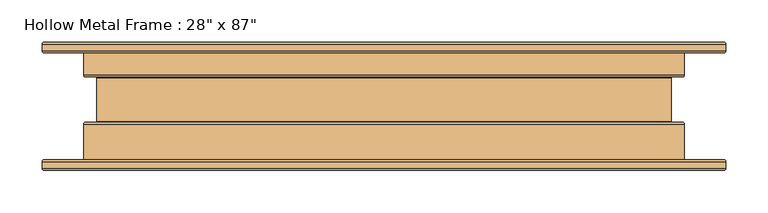
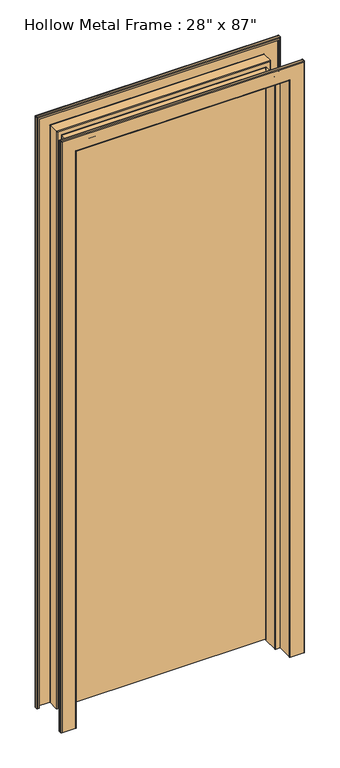
"""IFC4 building model written with IfcOpenShell, lengths in millimetres: door geometry."""

from ifc_helpers import new_model, si_unit, frame, origin, origin_with_axes, place, context, project, spatial, polyline, circle_curve, ellipse_curve, outline, extrude, source, transform, mapped, element, save
from ifc_brep_helpers import plane_surface, cylinder_surface, revolved_surface, advanced_brep


def door_6b69223f(model_context):
    return source(origin(), model_context, "Body", "SolidModel", [
        advanced_brep(
        [(-403.82825, -63.5635, 0.0), (-398.4625, -63.5635, 0.0), (-398.4625, -65.11925, 0.0), (-403.82825, -65.11925, 0.0), (-404.84425, -66.13525, 0.0), (-404.84425, -73.66, 0.0), (-403.82825, -74.676, 0.0), (-358.17175, -74.676, 0.0), (-357.15575, -73.66, 0.0), (-357.15575, -21.68525, 0.0), (-354.584, -19.1135, 0.0), (-342.29675, -19.1135, 0.0), (-341.28075, -18.0975, 0.0), (-341.28075, 33.6931, 0.0), (-342.29675, 34.7091, 0.0), (-354.584, 34.7091, 0.0), (-357.15575, 37.28085, 0.0), (-357.15575, 73.5965, 0.0), (-358.17175, 74.6125, 0.0), (-403.82825, 74.6125, 0.0), (-404.84425, 73.5965, 0.0), (-404.84425, 66.07175, 0.0), (-403.82825, 65.05575, 0.0), (-398.4625, 65.05575, 0.0), (-398.4625, 63.5, 0.0), (-403.82825, 63.5, 0.0), (-406.4, 66.07175, 0.0), (-406.4, 73.5965, 0.0), (-403.82825, 76.16825, 0.0), (-358.17175, 76.16825, 0.0), (-355.6, 73.5965, 0.0), (-355.6, 37.28085, 0.0), (-354.584, 36.26485, 0.0), (-342.29675, 36.26485, 0.0), (-339.725, 33.6931, 0.0), (-339.725, -18.0975, 0.0), (-342.29675, -20.66925, 0.0), (-354.584, -20.66925, 0.0), (-355.6, -21.68525, 0.0), (-355.6, -73.66, 0.0), (-358.17175, -76.23175, 0.0), (-403.82825, -76.23175, 0.0), (-406.4, -73.66, 0.0), (-406.4, -66.13525, 0.0), (-406.4, -66.13525, 2082.8000001), (-403.82825, -63.5635, 2080.2282501), (-406.4, -73.66, 2082.8000001), (-403.82825, -76.23175, 2080.2282501), (-358.17175, -76.23175, 2034.5717501), (358.17175, -76.23175, 2034.5717501), (358.17175, -76.23175, 0.0), (403.82825, -76.23175, 0.0), (403.82825, -76.23175, 2080.2282501), (-355.6, -73.66, 2032.0000001), (-355.6, -21.68525, 2032.0000001), (-354.584, -20.66925, 2030.9840001), (-342.29675, -20.66925, 2018.6967501), (342.29675, -20.66925, 2018.6967501), (342.29675, -20.66925, 0.0), (354.584, -20.66925, 0.0), (354.584, -20.66925, 2030.9840001), (-339.725, -18.0975, 2016.1250001), (-339.725, 33.6931, 2016.1250001), (-342.29675, 36.26485, 2018.6967501), (-354.584, 36.26485, 2030.9840001), (354.584, 36.26485, 2030.9840001), (354.584, 36.26485, 0.0), (342.29675, 36.26485, 0.0), (342.29675, 36.26485, 2018.6967501), (-355.6, 37.28085, 2032.0000001), (-355.6, 73.5965, 2032.0000001), (-358.17175, 76.16825, 2034.5717501), (-403.82825, 76.16825, 2080.2282501), (403.82825, 76.16825, 2080.2282501), (403.82825, 76.16825, 0.0), (358.17175, 76.16825, 0.0), (358.17175, 76.16825, 2034.5717501), (-406.4, 73.5965, 2082.8000001), (-406.4, 66.07175, 2082.8000001), (-403.82825, 63.5, 2080.2282501), (-398.4625, 63.5, 2074.8625001), (398.4625, 63.5, 2074.8625001), (398.4625, 63.5, 0.0), (403.82825, 63.5, 0.0), (403.82825, 63.5, 2080.2282501), (-398.4625, 65.05575, 2074.8625001), (-403.82825, 65.05575, 2080.2282501), (403.82825, 65.05575, 2080.2282501), (403.82825, 65.05575, 0.0), (398.4625, 65.05575, 0.0), (398.4625, 65.05575, 2074.8625001), (-404.84425, 66.07175, 2081.2442501), (-404.84425, 73.5965, 2081.2442501), (-403.82825, 74.6125, 2080.2282501), (-358.17175, 74.6125, 2034.5717501), (358.17175, 74.6125, 2034.5717501), (358.17175, 74.6125, 0.0), (403.82825, 74.6125, 0.0), (403.82825, 74.6125, 2080.2282501), (-357.15575, 73.5965, 2033.5557501), (-357.15575, 37.28085, 2033.5557501), (-354.584, 34.7091, 2030.9840001), (-342.29675, 34.7091, 2018.6967501), (342.29675, 34.7091, 2018.6967501), (342.29675, 34.7091, 0.0), (354.584, 34.7091, 0.0), (354.584, 34.7091, 2030.9840001), (-341.28075, 33.6931, 2017.6807501), (-341.28075, -18.0975, 2017.6807501), (-342.29675, -19.1135, 2018.6967501), (-354.584, -19.1135, 2030.9840001), (354.584, -19.1135, 2030.9840001), (354.584, -19.1135, 0.0), (342.29675, -19.1135, 0.0), (342.29675, -19.1135, 2018.6967501), (-357.15575, -21.68525, 2033.5557501), (-357.15575, -73.66, 2033.5557501), (-358.17175, -74.676, 2034.5717501), (-403.82825, -74.676, 2080.2282501), (403.82825, -74.676, 2080.2282501), (403.82825, -74.676, 0.0), (358.17175, -74.676, 0.0), (358.17175, -74.676, 2034.5717501), (-404.84425, -73.66, 2081.2442501), (-404.84425, -66.13525, 2081.2442501), (-403.82825, -65.11925, 2080.2282501), (-398.4625, -65.11925, 2074.8625001), (398.4625, -65.11925, 2074.8625001), (398.4625, -65.11925, 0.0), (403.82825, -65.11925, 0.0), (403.82825, -65.11925, 2080.2282501), (-398.4625, -63.5635, 2074.8625001), (403.82825, -63.5635, 2080.2282501), (403.82825, -63.5635, 0.0), (398.4625, -63.5635, 0.0), (398.4625, -63.5635, 2074.8625001), (406.4, -66.13525, 2082.8000001), (406.4, -73.66, 2082.8000001), (355.6, -73.66, 2032.0000001), (355.6, -21.68525, 2032.0000001), (339.725, -18.0975, 2016.1250001), (339.725, 33.6931, 2016.1250001), (355.6, 37.28085, 2032.0000001), (355.6, 73.5965, 2032.0000001), (406.4, 73.5965, 2082.8000001), (406.4, 66.07175, 2082.8000001), (404.84425, 66.07175, 2081.2442501), (404.84425, 73.5965, 2081.2442501), (357.15575, 73.5965, 2033.5557501), (357.15575, 37.28085, 2033.5557501), (341.28075, 33.6931, 2017.6807501), (341.28075, -18.0975, 2017.6807501), (357.15575, -21.68525, 2033.5557501), (357.15575, -73.66, 2033.5557501), (404.84425, -73.66, 2081.2442501), (404.84425, -66.13525, 2081.2442501), (406.4, -66.13525, 0.0), (406.4, -73.66, 0.0), (355.6, -73.66, 0.0), (355.6, -21.68525, 0.0), (339.725, -18.0975, 0.0), (339.725, 33.6931, 0.0), (355.6, 37.28085, 0.0), (355.6, 73.5965, 0.0), (406.4, 73.5965, 0.0), (406.4, 66.07175, 0.0), (404.84425, 66.07175, 0.0), (404.84425, 73.5965, 0.0), (357.15575, 73.5965, 0.0), (357.15575, 37.28085, 0.0), (341.28075, 33.6931, 0.0), (341.28075, -18.0975, 0.0), (357.15575, -21.68525, 0.0), (357.15575, -73.66, 0.0), (404.84425, -73.66, 0.0), (404.84425, -66.13525, 0.0)],
        [
            (0, 1),
            (1, 2),
            (2, 3),
            (3, 4, circle_curve(frame((-403.82825, -66.13525, 0.0), z_axis=(0.0, 0.0, 1.0), x_axis=(0.0, 1.0, 0.0)), 1.016)),
            (4, 5),
            (5, 6, circle_curve(frame((-403.82825, -73.66, 0.0), z_axis=(0.0, 0.0, 1.0), x_axis=(0.0, 1.0, 0.0)), 1.016)),
            (6, 7),
            (7, 8, circle_curve(frame((-358.17175, -73.66, 0.0), z_axis=(0.0, 0.0, 1.0), x_axis=(0.0, 1.0, 0.0)), 1.016)),
            (8, 9),
            (9, 10, circle_curve(frame((-354.584, -21.68525, 0.0), z_axis=(0.0, 0.0, -1.0), x_axis=(0.0, 1.0, 0.0)), 2.57175)),
            (10, 11),
            (11, 12, circle_curve(frame((-342.29675, -18.0975, 0.0), z_axis=(0.0, 0.0, 1.0), x_axis=(0.0, 1.0, 0.0)), 1.016)),
            (12, 13),
            (13, 14, circle_curve(frame((-342.29675, 33.6931, 0.0), z_axis=(0.0, 0.0, 1.0), x_axis=(0.0, 1.0, 0.0)), 1.016)),
            (14, 15),
            (15, 16, circle_curve(frame((-354.584, 37.28085, 0.0), z_axis=(0.0, 0.0, -1.0), x_axis=(0.0, 1.0, 0.0)), 2.57175)),
            (16, 17),
            (17, 18, circle_curve(frame((-358.17175, 73.5965, 0.0), z_axis=(0.0, 0.0, 1.0), x_axis=(0.0, 1.0, 0.0)), 1.016)),
            (18, 19),
            (19, 20, circle_curve(frame((-403.82825, 73.5965, 0.0), z_axis=(0.0, 0.0, 1.0), x_axis=(0.0, 1.0, 0.0)), 1.016)),
            (20, 21),
            (21, 22, circle_curve(frame((-403.82825, 66.07175, 0.0), z_axis=(0.0, 0.0, 1.0), x_axis=(0.0, 1.0, 0.0)), 1.016)),
            (22, 23),
            (23, 24),
            (24, 25),
            (25, 26, circle_curve(frame((-403.82825, 66.07175, 0.0), z_axis=(0.0, 0.0, -1.0), x_axis=(0.0, 1.0, 0.0)), 2.57175)),
            (26, 27),
            (27, 28, circle_curve(frame((-403.82825, 73.5965, 0.0), z_axis=(0.0, 0.0, -1.0), x_axis=(0.0, 1.0, 0.0)), 2.57175)),
            (28, 29),
            (29, 30, circle_curve(frame((-358.17175, 73.5965, 0.0), z_axis=(0.0, 0.0, -1.0), x_axis=(0.0, 1.0, 0.0)), 2.57175)),
            (30, 31),
            (31, 32, circle_curve(frame((-354.584, 37.28085, 0.0), z_axis=(0.0, 0.0, 1.0), x_axis=(0.0, 1.0, 0.0)), 1.016)),
            (32, 33),
            (33, 34, circle_curve(frame((-342.29675, 33.6931, 0.0), z_axis=(0.0, 0.0, -1.0), x_axis=(0.0, 1.0, 0.0)), 2.57175)),
            (34, 35),
            (35, 36, circle_curve(frame((-342.29675, -18.0975, 0.0), z_axis=(0.0, 0.0, -1.0), x_axis=(0.0, 1.0, 0.0)), 2.57175)),
            (36, 37),
            (37, 38, circle_curve(frame((-354.584, -21.68525, 0.0), z_axis=(0.0, 0.0, 1.0), x_axis=(0.0, 1.0, 0.0)), 1.016)),
            (38, 39),
            (39, 40, circle_curve(frame((-358.17175, -73.66, 0.0), z_axis=(0.0, 0.0, -1.0), x_axis=(0.0, 1.0, 0.0)), 2.57175)),
            (40, 41),
            (41, 42, circle_curve(frame((-403.82825, -73.66, 0.0), z_axis=(0.0, 0.0, -1.0), x_axis=(0.0, 1.0, 0.0)), 2.57175)),
            (42, 43),
            (43, 0, circle_curve(frame((-403.82825, -66.13525, 0.0), z_axis=(0.0, 0.0, -1.0), x_axis=(0.0, 1.0, 0.0)), 2.57175)),
            (43, 44),
            (44, 45, ellipse_curve(frame((-403.82825, -66.13525, 2080.2282501), z_axis=(-0.7071067811865475, 0.0, -0.7071067811865475), x_axis=(0.7071067811865474, 0.0, -0.7071067811865476)), 3.6370037, 2.57175)),
            (45, 0),
            (42, 46),
            (46, 44),
            (41, 47),
            (47, 46, ellipse_curve(frame((-403.82825, -73.66, 2080.2282501), z_axis=(-0.7071067811865475, 0.0, -0.7071067811865475), x_axis=(0.7071067811865474, 0.0, -0.7071067811865476)), 3.6370037, 2.57175)),
            (40, 48),
            (48, 49),
            (49, 50),
            (50, 51),
            (51, 52),
            (52, 47),
            (39, 53),
            (53, 48, ellipse_curve(frame((-358.17175, -73.66, 2034.5717501), z_axis=(-0.7071067811865475, 0.0, -0.7071067811865475), x_axis=(0.7071067811865474, 0.0, -0.7071067811865476)), 3.6370037, 2.57175)),
            (38, 54),
            (54, 53),
            (37, 55),
            (55, 54, ellipse_curve(frame((-354.584, -21.68525, 2030.9840001), z_axis=(0.7071067811865475, 0.0, 0.7071067811865475), x_axis=(-0.7071067811865474, 0.0, 0.7071067811865476)), 1.436841, 1.016)),
            (36, 56),
            (56, 57),
            (57, 58),
            (58, 59),
            (59, 60),
            (60, 55),
            (35, 61),
            (61, 56, ellipse_curve(frame((-342.29675, -18.0975, 2018.6967501), z_axis=(-0.7071067811865475, 0.0, -0.7071067811865475), x_axis=(0.7071067811865474, 0.0, -0.7071067811865476)), 3.6370037, 2.57175)),
            (34, 62),
            (62, 61),
            (33, 63),
            (63, 62, ellipse_curve(frame((-342.29675, 33.6931, 2018.6967501), z_axis=(-0.7071067811865475, 0.0, -0.7071067811865475), x_axis=(0.7071067811865474, 0.0, -0.7071067811865476)), 3.6370037, 2.57175)),
            (32, 64),
            (64, 65),
            (65, 66),
            (66, 67),
            (67, 68),
            (68, 63),
            (31, 69),
            (69, 64, ellipse_curve(frame((-354.584, 37.28085, 2030.9840001), z_axis=(0.7071067811865475, 0.0, 0.7071067811865475), x_axis=(-0.7071067811865474, 0.0, 0.7071067811865476)), 1.436841, 1.016)),
            (30, 70),
            (70, 69),
            (29, 71),
            (71, 70, ellipse_curve(frame((-358.17175, 73.5965, 2034.5717501), z_axis=(-0.7071067811865475, 0.0, -0.7071067811865475), x_axis=(0.7071067811865474, 0.0, -0.7071067811865476)), 3.6370037, 2.57175)),
            (28, 72),
            (72, 73),
            (73, 74),
            (74, 75),
            (75, 76),
            (76, 71),
            (27, 77),
            (77, 72, ellipse_curve(frame((-403.82825, 73.5965, 2080.2282501), z_axis=(-0.7071067811865475, 0.0, -0.7071067811865475), x_axis=(0.7071067811865474, 0.0, -0.7071067811865476)), 3.6370037, 2.57175)),
            (26, 78),
            (78, 77),
            (25, 79),
            (79, 78, ellipse_curve(frame((-403.82825, 66.07175, 2080.2282501), z_axis=(-0.7071067811865475, 0.0, -0.7071067811865475), x_axis=(0.7071067811865474, 0.0, -0.7071067811865476)), 3.6370037, 2.57175)),
            (24, 80),
            (80, 81),
            (81, 82),
            (82, 83),
            (83, 84),
            (84, 79),
            (23, 85),
            (85, 80),
            (22, 86),
            (86, 87),
            (87, 88),
            (88, 89),
            (89, 90),
            (90, 85),
            (21, 91),
            (91, 86, ellipse_curve(frame((-403.82825, 66.07175, 2080.2282501), z_axis=(0.7071067811865475, 0.0, 0.7071067811865475), x_axis=(-0.7071067811865474, 0.0, 0.7071067811865476)), 1.436841, 1.016)),
            (20, 92),
            (92, 91),
            (19, 93),
            (93, 92, ellipse_curve(frame((-403.82825, 73.5965, 2080.2282501), z_axis=(0.7071067811865475, 0.0, 0.7071067811865475), x_axis=(-0.7071067811865474, 0.0, 0.7071067811865476)), 1.436841, 1.016)),
            (18, 94),
            (94, 95),
            (95, 96),
            (96, 97),
            (97, 98),
            (98, 93),
            (17, 99),
            (99, 94, ellipse_curve(frame((-358.17175, 73.5965, 2034.5717501), z_axis=(0.7071067811865475, 0.0, 0.7071067811865475), x_axis=(-0.7071067811865474, 0.0, 0.7071067811865476)), 1.436841, 1.016)),
            (16, 100),
            (100, 99),
            (15, 101),
            (101, 100, ellipse_curve(frame((-354.584, 37.28085, 2030.9840001), z_axis=(-0.7071067811865475, 0.0, -0.7071067811865475), x_axis=(0.7071067811865474, 0.0, -0.7071067811865476)), 3.6370037, 2.57175)),
            (14, 102),
            (102, 103),
            (103, 104),
            (104, 105),
            (105, 106),
            (106, 101),
            (13, 107),
            (107, 102, ellipse_curve(frame((-342.29675, 33.6931, 2018.6967501), z_axis=(0.7071067811865475, 0.0, 0.7071067811865475), x_axis=(-0.7071067811865474, 0.0, 0.7071067811865476)), 1.436841, 1.016)),
            (12, 108),
            (108, 107),
            (11, 109),
            (109, 108, ellipse_curve(frame((-342.29675, -18.0975, 2018.6967501), z_axis=(0.7071067811865475, 0.0, 0.7071067811865475), x_axis=(-0.7071067811865474, 0.0, 0.7071067811865476)), 1.436841, 1.016)),
            (10, 110),
            (110, 111),
            (111, 112),
            (112, 113),
            (113, 114),
            (114, 109),
            (9, 115),
            (115, 110, ellipse_curve(frame((-354.584, -21.68525, 2030.9840001), z_axis=(-0.7071067811865475, 0.0, -0.7071067811865475), x_axis=(0.7071067811865474, 0.0, -0.7071067811865476)), 3.6370037, 2.57175)),
            (8, 116),
            (116, 115),
            (7, 117),
            (117, 116, ellipse_curve(frame((-358.17175, -73.66, 2034.5717501), z_axis=(0.7071067811865475, 0.0, 0.7071067811865475), x_axis=(-0.7071067811865474, 0.0, 0.7071067811865476)), 1.436841, 1.016)),
            (6, 118),
            (118, 119),
            (119, 120),
            (120, 121),
            (121, 122),
            (122, 117),
            (5, 123),
            (123, 118, ellipse_curve(frame((-403.82825, -73.66, 2080.2282501), z_axis=(0.7071067811865475, 0.0, 0.7071067811865475), x_axis=(-0.7071067811865474, 0.0, 0.7071067811865476)), 1.436841, 1.016)),
            (4, 124),
            (124, 123),
            (3, 125),
            (125, 124, ellipse_curve(frame((-403.82825, -66.13525, 2080.2282501), z_axis=(0.7071067811865475, 0.0, 0.7071067811865475), x_axis=(-0.7071067811865474, 0.0, 0.7071067811865476)), 1.436841, 1.016)),
            (2, 126),
            (126, 127),
            (127, 128),
            (128, 129),
            (129, 130),
            (130, 125),
            (1, 131),
            (131, 126),
            (45, 132),
            (132, 133),
            (133, 134),
            (134, 135),
            (135, 131),
            (44, 136),
            (136, 132, ellipse_curve(frame((403.82825, -66.13525, 2080.2282501), z_axis=(-0.7071067811865475, 0.0, 0.7071067811865475), x_axis=(-0.7071067811865476, 0.0, -0.7071067811865474)), 3.6370037, 2.57175)),
            (46, 137),
            (137, 136),
            (52, 137, ellipse_curve(frame((403.82825, -73.66, 2080.2282501), z_axis=(-0.7071067811865475, 0.0, 0.7071067811865475), x_axis=(-0.7071067811865476, 0.0, -0.7071067811865474)), 3.6370037, 2.57175)),
            (53, 138),
            (138, 49, ellipse_curve(frame((358.17175, -73.66, 2034.5717501), z_axis=(-0.7071067811865475, 0.0, 0.7071067811865475), x_axis=(-0.7071067811865476, 0.0, -0.7071067811865474)), 3.6370037, 2.57175)),
            (54, 139),
            (139, 138),
            (60, 139, ellipse_curve(frame((354.584, -21.68525, 2030.9840001), z_axis=(0.7071067811865475, 0.0, -0.7071067811865475), x_axis=(0.7071067811865476, 0.0, 0.7071067811865474)), 1.436841, 1.016)),
            (61, 140),
            (140, 57, ellipse_curve(frame((342.29675, -18.0975, 2018.6967501), z_axis=(-0.7071067811865475, 0.0, 0.7071067811865475), x_axis=(-0.7071067811865476, 0.0, -0.7071067811865474)), 3.6370037, 2.57175)),
            (62, 141),
            (141, 140),
            (68, 141, ellipse_curve(frame((342.29675, 33.6931, 2018.6967501), z_axis=(-0.7071067811865475, 0.0, 0.7071067811865475), x_axis=(-0.7071067811865476, 0.0, -0.7071067811865474)), 3.6370037, 2.57175)),
            (69, 142),
            (142, 65, ellipse_curve(frame((354.584, 37.28085, 2030.9840001), z_axis=(0.7071067811865475, 0.0, -0.7071067811865475), x_axis=(0.7071067811865476, 0.0, 0.7071067811865474)), 1.436841, 1.016)),
            (70, 143),
            (143, 142),
            (76, 143, ellipse_curve(frame((358.17175, 73.5965, 2034.5717501), z_axis=(-0.7071067811865475, 0.0, 0.7071067811865475), x_axis=(-0.7071067811865476, 0.0, -0.7071067811865474)), 3.6370037, 2.57175)),
            (77, 144),
            (144, 73, ellipse_curve(frame((403.82825, 73.5965, 2080.2282501), z_axis=(-0.7071067811865475, 0.0, 0.7071067811865475), x_axis=(-0.7071067811865476, 0.0, -0.7071067811865474)), 3.6370037, 2.57175)),
            (78, 145),
            (145, 144),
            (84, 145, ellipse_curve(frame((403.82825, 66.07175, 2080.2282501), z_axis=(-0.7071067811865475, 0.0, 0.7071067811865475), x_axis=(-0.7071067811865476, 0.0, -0.7071067811865474)), 3.6370037, 2.57175)),
            (90, 81),
            (91, 146),
            (146, 87, ellipse_curve(frame((403.82825, 66.07175, 2080.2282501), z_axis=(0.7071067811865475, 0.0, -0.7071067811865475), x_axis=(0.7071067811865476, 0.0, 0.7071067811865474)), 1.436841, 1.016)),
            (92, 147),
            (147, 146),
            (98, 147, ellipse_curve(frame((403.82825, 73.5965, 2080.2282501), z_axis=(0.7071067811865475, 0.0, -0.7071067811865475), x_axis=(0.7071067811865476, 0.0, 0.7071067811865474)), 1.436841, 1.016)),
            (99, 148),
            (148, 95, ellipse_curve(frame((358.17175, 73.5965, 2034.5717501), z_axis=(0.7071067811865475, 0.0, -0.7071067811865475), x_axis=(0.7071067811865476, 0.0, 0.7071067811865474)), 1.436841, 1.016)),
            (100, 149),
            (149, 148),
            (106, 149, ellipse_curve(frame((354.584, 37.28085, 2030.9840001), z_axis=(-0.7071067811865475, 0.0, 0.7071067811865475), x_axis=(-0.7071067811865476, 0.0, -0.7071067811865474)), 3.6370037, 2.57175)),
            (107, 150),
            (150, 103, ellipse_curve(frame((342.29675, 33.6931, 2018.6967501), z_axis=(0.7071067811865475, 0.0, -0.7071067811865475), x_axis=(0.7071067811865476, 0.0, 0.7071067811865474)), 1.436841, 1.016)),
            (108, 151),
            (151, 150),
            (114, 151, ellipse_curve(frame((342.29675, -18.0975, 2018.6967501), z_axis=(0.7071067811865475, 0.0, -0.7071067811865475), x_axis=(0.7071067811865476, 0.0, 0.7071067811865474)), 1.436841, 1.016)),
            (115, 152),
            (152, 111, ellipse_curve(frame((354.584, -21.68525, 2030.9840001), z_axis=(-0.7071067811865475, 0.0, 0.7071067811865475), x_axis=(-0.7071067811865476, 0.0, -0.7071067811865474)), 3.6370037, 2.57175)),
            (116, 153),
            (153, 152),
            (122, 153, ellipse_curve(frame((358.17175, -73.66, 2034.5717501), z_axis=(0.7071067811865475, 0.0, -0.7071067811865475), x_axis=(0.7071067811865476, 0.0, 0.7071067811865474)), 1.436841, 1.016)),
            (123, 154),
            (154, 119, ellipse_curve(frame((403.82825, -73.66, 2080.2282501), z_axis=(0.7071067811865475, 0.0, -0.7071067811865475), x_axis=(0.7071067811865476, 0.0, 0.7071067811865474)), 1.436841, 1.016)),
            (124, 155),
            (155, 154),
            (130, 155, ellipse_curve(frame((403.82825, -66.13525, 2080.2282501), z_axis=(0.7071067811865475, 0.0, -0.7071067811865475), x_axis=(0.7071067811865476, 0.0, 0.7071067811865474)), 1.436841, 1.016)),
            (135, 127),
            (133, 156, circle_curve(frame((403.82825, -66.13525, 0.0), z_axis=(0.0, 0.0, -1.0), x_axis=(0.0, 1.0, 0.0)), 2.57175)),
            (156, 157),
            (157, 51, circle_curve(frame((403.82825, -73.66, 0.0), z_axis=(0.0, 0.0, -1.0), x_axis=(0.0, 1.0, 0.0)), 2.57175)),
            (50, 158, circle_curve(frame((358.17175, -73.66, 0.0), z_axis=(0.0, 0.0, -1.0), x_axis=(0.0, 1.0, 0.0)), 2.57175)),
            (158, 159),
            (159, 59, circle_curve(frame((354.584, -21.68525, 0.0), z_axis=(0.0, 0.0, 1.0), x_axis=(0.0, 1.0, 0.0)), 1.016)),
            (58, 160, circle_curve(frame((342.29675, -18.0975, 0.0), z_axis=(0.0, 0.0, -1.0), x_axis=(0.0, 1.0, 0.0)), 2.57175)),
            (160, 161),
            (161, 67, circle_curve(frame((342.29675, 33.6931, 0.0), z_axis=(0.0, 0.0, -1.0), x_axis=(0.0, 1.0, 0.0)), 2.57175)),
            (66, 162, circle_curve(frame((354.584, 37.28085, 0.0), z_axis=(0.0, 0.0, 1.0), x_axis=(0.0, 1.0, 0.0)), 1.016)),
            (162, 163),
            (163, 75, circle_curve(frame((358.17175, 73.5965, 0.0), z_axis=(0.0, 0.0, -1.0), x_axis=(0.0, 1.0, 0.0)), 2.57175)),
            (74, 164, circle_curve(frame((403.82825, 73.5965, 0.0), z_axis=(0.0, 0.0, -1.0), x_axis=(0.0, 1.0, 0.0)), 2.57175)),
            (164, 165),
            (165, 83, circle_curve(frame((403.82825, 66.07175, 0.0), z_axis=(0.0, 0.0, -1.0), x_axis=(0.0, 1.0, 0.0)), 2.57175)),
            (82, 89),
            (88, 166, circle_curve(frame((403.82825, 66.07175, 0.0), z_axis=(0.0, 0.0, 1.0), x_axis=(0.0, 1.0, 0.0)), 1.016)),
            (166, 167),
            (167, 97, circle_curve(frame((403.82825, 73.5965, 0.0), z_axis=(0.0, 0.0, 1.0), x_axis=(0.0, 1.0, 0.0)), 1.016)),
            (96, 168, circle_curve(frame((358.17175, 73.5965, 0.0), z_axis=(0.0, 0.0, 1.0), x_axis=(0.0, 1.0, 0.0)), 1.016)),
            (168, 169),
            (169, 105, circle_curve(frame((354.584, 37.28085, 0.0), z_axis=(0.0, 0.0, -1.0), x_axis=(0.0, 1.0, 0.0)), 2.57175)),
            (104, 170, circle_curve(frame((342.29675, 33.6931, 0.0), z_axis=(0.0, 0.0, 1.0), x_axis=(0.0, 1.0, 0.0)), 1.016)),
            (170, 171),
            (171, 113, circle_curve(frame((342.29675, -18.0975, 0.0), z_axis=(0.0, 0.0, 1.0), x_axis=(0.0, 1.0, 0.0)), 1.016)),
            (112, 172, circle_curve(frame((354.584, -21.68525, 0.0), z_axis=(0.0, 0.0, -1.0), x_axis=(0.0, 1.0, 0.0)), 2.57175)),
            (172, 173),
            (173, 121, circle_curve(frame((358.17175, -73.66, 0.0), z_axis=(0.0, 0.0, 1.0), x_axis=(0.0, 1.0, 0.0)), 1.016)),
            (120, 174, circle_curve(frame((403.82825, -73.66, 0.0), z_axis=(0.0, 0.0, 1.0), x_axis=(0.0, 1.0, 0.0)), 1.016)),
            (174, 175),
            (175, 129, circle_curve(frame((403.82825, -66.13525, 0.0), z_axis=(0.0, 0.0, 1.0), x_axis=(0.0, 1.0, 0.0)), 1.016)),
            (128, 134),
            (136, 156),
            (137, 157),
            (138, 158),
            (139, 159),
            (140, 160),
            (141, 161),
            (142, 162),
            (143, 163),
            (144, 164),
            (145, 165),
            (146, 166),
            (147, 167),
            (148, 168),
            (149, 169),
            (150, 170),
            (151, 171),
            (152, 172),
            (153, 173),
            (154, 174),
            (155, 175),
        ],
        [
            plane_surface(frame((-366.7125, 63.5, 0.0), z_axis=(0.0, 0.0, -1.0), x_axis=(1.0, 0.0, 0.0))),
            cylinder_surface(frame((-403.82825, -66.13525, 0.0), z_axis=(0.0, 0.0, -1.0), x_axis=(0.0, 1.0, 0.0)), 2.57175),
            plane_surface(frame((-406.4, -66.13525, 0.0), z_axis=(-1.0, 0.0, 0.0), x_axis=(0.0, 0.0, 1.0))),
            cylinder_surface(frame((-403.82825, -73.66, 0.0), z_axis=(0.0, 0.0, -1.0), x_axis=(0.0, 1.0, 0.0)), 2.57175),
            plane_surface(frame((-403.82825, -76.23175, 0.0), z_axis=(0.0, -1.0, 0.0), x_axis=(0.0, 0.0, 1.0))),
            cylinder_surface(frame((-358.17175, -73.66, 0.0), z_axis=(0.0, 0.0, -1.0), x_axis=(0.0, 1.0, 0.0)), 2.57175),
            plane_surface(frame((-355.6, -73.66, 0.0), z_axis=(1.0, 0.0, 0.0), x_axis=(0.0, 0.0, 1.0))),
            revolved_surface(polyline([(-354.584, -20.669249999999998, 2032.0000001145868), (-354.584, -20.669249999999998, 0.0)]), (-354.584, -21.68525, 0.0), (0.0, 0.0, 1.0)),
            plane_surface(frame((-354.584, -20.66925, 0.0), z_axis=(0.0, -1.0, 0.0), x_axis=(0.0, 0.0, 1.0))),
            cylinder_surface(frame((-342.29675, -18.0975, 0.0), z_axis=(0.0, 0.0, -1.0), x_axis=(0.0, 1.0, 0.0)), 2.57175),
            plane_surface(frame((-339.725, -18.0975, 0.0), z_axis=(1.0, 0.0, 0.0), x_axis=(0.0, 0.0, 1.0))),
            cylinder_surface(frame((-342.29675, 33.6931, 0.0), z_axis=(0.0, 0.0, -1.0), x_axis=(0.0, 1.0, 0.0)), 2.57175),
            plane_surface(frame((-342.29675, 36.26485, 0.0), z_axis=(0.0, 1.0, 0.0), x_axis=(0.0, 0.0, 1.0))),
            revolved_surface(polyline([(-354.584, 38.29685, 2032.0000001145868), (-354.584, 38.29685, 0.0)]), (-354.584, 37.28085, 0.0), (0.0, 0.0, 1.0)),
            plane_surface(frame((-355.6, 37.28085, 0.0), z_axis=(1.0, 0.0, 0.0), x_axis=(0.0, 0.0, 1.0))),
            cylinder_surface(frame((-358.17175, 73.5965, 0.0), z_axis=(0.0, 0.0, -1.0), x_axis=(0.0, 1.0, 0.0)), 2.57175),
            plane_surface(frame((-358.17175, 76.16825, 0.0), z_axis=(0.0, 1.0, 0.0), x_axis=(0.0, 0.0, 1.0))),
            cylinder_surface(frame((-403.82825, 73.5965, 0.0), z_axis=(0.0, 0.0, -1.0), x_axis=(0.0, 1.0, 0.0)), 2.57175),
            plane_surface(frame((-406.4, 73.5965, 0.0), z_axis=(-1.0, 0.0, 0.0), x_axis=(0.0, 0.0, 1.0))),
            cylinder_surface(frame((-403.82825, 66.07175, 0.0), z_axis=(0.0, 0.0, -1.0), x_axis=(0.0, 1.0, 0.0)), 2.57175),
            plane_surface(frame((-403.82825, 63.5, 0.0), z_axis=(0.0, -1.0, 0.0), x_axis=(0.0, 0.0, 1.0))),
            plane_surface(frame((-398.4625, 63.5, 0.0), z_axis=(1.0, 0.0, 0.0), x_axis=(0.0, 0.0, 1.0))),
            plane_surface(frame((-398.4625, 65.05575, 0.0), z_axis=(0.0, 1.0, 0.0), x_axis=(0.0, 0.0, 1.0))),
            revolved_surface(polyline([(-403.82825, 67.08775, 2081.244250114587), (-403.82825, 67.08775, 0.0)]), (-403.82825, 66.07175, 0.0), (0.0, 0.0, 1.0)),
            plane_surface(frame((-404.84425, 66.07175, 0.0), z_axis=(1.0, 0.0, 0.0), x_axis=(0.0, 0.0, 1.0))),
            revolved_surface(polyline([(-403.82825, 74.61250000000001, 2081.244250114587), (-403.82825, 74.61250000000001, 0.0)]), (-403.82825, 73.5965, 0.0), (0.0, 0.0, 1.0)),
            plane_surface(frame((-403.82825, 74.6125, 0.0), z_axis=(0.0, -1.0, 0.0), x_axis=(0.0, 0.0, 1.0))),
            revolved_surface(polyline([(-358.17175, 74.61250000000001, 2035.5877501145867), (-358.17175, 74.61250000000001, 0.0)]), (-358.17175, 73.5965, 0.0), (0.0, 0.0, 1.0)),
            plane_surface(frame((-357.15575, 73.5965, 0.0), z_axis=(-1.0, 0.0, 0.0), x_axis=(0.0, 0.0, 1.0))),
            cylinder_surface(frame((-354.584, 37.28085, 0.0), z_axis=(0.0, 0.0, -1.0), x_axis=(0.0, 1.0, 0.0)), 2.57175),
            plane_surface(frame((-354.584, 34.7091, 0.0), z_axis=(0.0, -1.0, 0.0), x_axis=(0.0, 0.0, 1.0))),
            revolved_surface(polyline([(-342.29675, 34.7091, 2019.7127501145867), (-342.29675, 34.7091, 0.0)]), (-342.29675, 33.6931, 0.0), (0.0, 0.0, 1.0)),
            plane_surface(frame((-341.28075, 33.6931, 0.0), z_axis=(-1.0, 0.0, 0.0), x_axis=(0.0, 0.0, 1.0))),
            revolved_surface(polyline([(-342.29675, -17.0815, 2019.7127501145867), (-342.29675, -17.0815, 0.0)]), (-342.29675, -18.0975, 0.0), (0.0, 0.0, 1.0)),
            plane_surface(frame((-342.29675, -19.1135, 0.0), z_axis=(0.0, 1.0, 0.0), x_axis=(0.0, 0.0, 1.0))),
            cylinder_surface(frame((-354.584, -21.68525, 0.0), z_axis=(0.0, 0.0, -1.0), x_axis=(0.0, 1.0, 0.0)), 2.57175),
            plane_surface(frame((-357.15575, -21.68525, 0.0), z_axis=(-1.0, 0.0, 0.0), x_axis=(0.0, 0.0, 1.0))),
            revolved_surface(polyline([(-358.17175, -72.64399999999999, 2035.5877501145867), (-358.17175, -72.64399999999999, 0.0)]), (-358.17175, -73.66, 0.0), (0.0, 0.0, 1.0)),
            plane_surface(frame((-358.17175, -74.676, 0.0), z_axis=(0.0, 1.0, 0.0), x_axis=(0.0, 0.0, 1.0))),
            revolved_surface(polyline([(-403.82825, -72.64399999999999, 2081.244250114587), (-403.82825, -72.64399999999999, 0.0)]), (-403.82825, -73.66, 0.0), (0.0, 0.0, 1.0)),
            plane_surface(frame((-404.84425, -73.66, 0.0), z_axis=(1.0, 0.0, 0.0), x_axis=(0.0, 0.0, 1.0))),
            revolved_surface(polyline([(-403.82825, -65.11925, 2081.244250114587), (-403.82825, -65.11925, 0.0)]), (-403.82825, -66.13525, 0.0), (0.0, 0.0, 1.0)),
            plane_surface(frame((-403.82825, -65.11925, 0.0), z_axis=(0.0, -1.0, 0.0), x_axis=(0.0, 0.0, 1.0))),
            plane_surface(frame((-398.4625, -65.11925, 0.0), z_axis=(1.0, 0.0, 0.0), x_axis=(0.0, 0.0, 1.0))),
            plane_surface(frame((-398.4625, -63.5635, 0.0), z_axis=(0.0, 1.0, 0.0), x_axis=(0.0, 0.0, 1.0))),
            cylinder_surface(frame((-366.7125, -66.13525, 2080.2282501), z_axis=(-1.0, 0.0, 0.0), x_axis=(0.0, 1.0, 0.0)), 2.57175),
            plane_surface(frame((-406.4, -66.13525, 2082.8000001), z_axis=(0.0, 0.0, 1.0), x_axis=(1.0, 0.0, 0.0))),
            cylinder_surface(frame((-366.7125, -73.66, 2080.2282501), z_axis=(-1.0, 0.0, 0.0), x_axis=(0.0, 1.0, 0.0)), 2.57175),
            cylinder_surface(frame((-366.7125, -73.66, 2034.5717501), z_axis=(-1.0, 0.0, 0.0), x_axis=(0.0, 1.0, 0.0)), 2.57175),
            plane_surface(frame((-355.6, -73.66, 2032.0000001), z_axis=(0.0, 0.0, -1.0), x_axis=(1.0, 0.0, 0.0))),
            revolved_surface(polyline([(355.60000001458684, -20.669249999999998, 2030.9840001), (-355.60000001458684, -20.669249999999998, 2030.9840001)]), (-366.7125, -21.68525, 2030.9840001), (1.0, 0.0, 0.0)),
            cylinder_surface(frame((-366.7125, -18.0975, 2018.6967501), z_axis=(-1.0, 0.0, 0.0), x_axis=(0.0, 1.0, 0.0)), 2.57175),
            plane_surface(frame((-339.725, -18.0975, 2016.1250001), z_axis=(0.0, 0.0, -1.0), x_axis=(1.0, 0.0, 0.0))),
            cylinder_surface(frame((-366.7125, 33.6931, 2018.6967501), z_axis=(-1.0, 0.0, 0.0), x_axis=(0.0, 1.0, 0.0)), 2.57175),
            revolved_surface(polyline([(355.60000001458684, 38.29685, 2030.9840001), (-355.60000001458684, 38.29685, 2030.9840001)]), (-366.7125, 37.28085, 2030.9840001), (1.0, 0.0, 0.0)),
            plane_surface(frame((-355.6, 37.28085, 2032.0000001), z_axis=(0.0, 0.0, -1.0), x_axis=(1.0, 0.0, 0.0))),
            cylinder_surface(frame((-366.7125, 73.5965, 2034.5717501), z_axis=(-1.0, 0.0, 0.0), x_axis=(0.0, 1.0, 0.0)), 2.57175),
            cylinder_surface(frame((-366.7125, 73.5965, 2080.2282501), z_axis=(-1.0, 0.0, 0.0), x_axis=(0.0, 1.0, 0.0)), 2.57175),
            plane_surface(frame((-406.4, 73.5965, 2082.8000001), z_axis=(0.0, 0.0, 1.0), x_axis=(1.0, 0.0, 0.0))),
            cylinder_surface(frame((-366.7125, 66.07175, 2080.2282501), z_axis=(-1.0, 0.0, 0.0), x_axis=(0.0, 1.0, 0.0)), 2.57175),
            plane_surface(frame((-398.4625, 63.5, 2074.8625001), z_axis=(0.0, 0.0, -1.0), x_axis=(1.0, 0.0, 0.0))),
            revolved_surface(polyline([(404.8442500145869, 67.08775, 2080.2282501), (-404.84425001458686, 67.08775, 2080.2282501)]), (-366.7125, 66.07175, 2080.2282501), (1.0, 0.0, 0.0)),
            plane_surface(frame((-404.84425, 66.07175, 2081.2442501), z_axis=(0.0, 0.0, -1.0), x_axis=(1.0, 0.0, 0.0))),
            revolved_surface(polyline([(404.8442500145869, 74.61250000000001, 2080.2282501), (-404.84425001458686, 74.61250000000001, 2080.2282501)]), (-366.7125, 73.5965, 2080.2282501), (1.0, 0.0, 0.0)),
            revolved_surface(polyline([(359.18775001458687, 74.61250000000001, 2034.5717501), (-359.1877500145868, 74.61250000000001, 2034.5717501)]), (-366.7125, 73.5965, 2034.5717501), (1.0, 0.0, 0.0)),
            plane_surface(frame((-357.15575, 73.5965, 2033.5557501), z_axis=(0.0, 0.0, 1.0), x_axis=(1.0, 0.0, 0.0))),
            cylinder_surface(frame((-366.7125, 37.28085, 2030.9840001), z_axis=(-1.0, 0.0, 0.0), x_axis=(0.0, 1.0, 0.0)), 2.57175),
            revolved_surface(polyline([(343.31275001458687, 34.7091, 2018.6967501), (-343.3127500145868, 34.7091, 2018.6967501)]), (-366.7125, 33.6931, 2018.6967501), (1.0, 0.0, 0.0)),
            plane_surface(frame((-341.28075, 33.6931, 2017.6807501), z_axis=(0.0, 0.0, 1.0), x_axis=(1.0, 0.0, 0.0))),
            revolved_surface(polyline([(343.31275001458687, -17.0815, 2018.6967501), (-343.3127500145868, -17.0815, 2018.6967501)]), (-366.7125, -18.0975, 2018.6967501), (1.0, 0.0, 0.0)),
            cylinder_surface(frame((-366.7125, -21.68525, 2030.9840001), z_axis=(-1.0, 0.0, 0.0), x_axis=(0.0, 1.0, 0.0)), 2.57175),
            plane_surface(frame((-357.15575, -21.68525, 2033.5557501), z_axis=(0.0, 0.0, 1.0), x_axis=(1.0, 0.0, 0.0))),
            revolved_surface(polyline([(359.18775001458687, -72.64399999999999, 2034.5717501), (-359.1877500145868, -72.64399999999999, 2034.5717501)]), (-366.7125, -73.66, 2034.5717501), (1.0, 0.0, 0.0)),
            revolved_surface(polyline([(404.8442500145869, -72.64399999999999, 2080.2282501), (-404.84425001458686, -72.64399999999999, 2080.2282501)]), (-366.7125, -73.66, 2080.2282501), (1.0, 0.0, 0.0)),
            plane_surface(frame((-404.84425, -73.66, 2081.2442501), z_axis=(0.0, 0.0, -1.0), x_axis=(1.0, 0.0, 0.0))),
            revolved_surface(polyline([(404.8442500145869, -65.11925, 2080.2282501), (-404.84425001458686, -65.11925, 2080.2282501)]), (-366.7125, -66.13525, 2080.2282501), (1.0, 0.0, 0.0)),
            plane_surface(frame((-398.4625, -65.11925, 2074.8625001), z_axis=(0.0, 0.0, -1.0), x_axis=(1.0, 0.0, 0.0))),
            plane_surface(frame((366.7125, 63.5, 0.0), z_axis=(0.0, 0.0, -1.0), x_axis=(-1.0, 0.0, 0.0))),
            cylinder_surface(frame((403.82825, -66.13525, 2043.1125001), z_axis=(0.0, 0.0, 1.0), x_axis=(0.0, 1.0, 0.0)), 2.57175),
            plane_surface(frame((406.4, -66.13525, 2082.8000001), z_axis=(1.0, 0.0, 0.0), x_axis=(0.0, 0.0, -1.0))),
            cylinder_surface(frame((403.82825, -73.66, 2043.1125001), z_axis=(0.0, 0.0, 1.0), x_axis=(0.0, 1.0, 0.0)), 2.57175),
            cylinder_surface(frame((358.17175, -73.66, 2043.1125001), z_axis=(0.0, 0.0, 1.0), x_axis=(0.0, 1.0, 0.0)), 2.57175),
            plane_surface(frame((355.6, -73.66, 2032.0000001), z_axis=(-1.0, 0.0, 0.0), x_axis=(0.0, 0.0, -1.0))),
            revolved_surface(polyline([(354.584, -20.669249999999998, 0.0), (354.584, -20.669249999999998, 2032.0000001145868)]), (354.584, -21.68525, 2043.1125001), (0.0, 0.0, -1.0)),
            cylinder_surface(frame((342.29675, -18.0975, 2043.1125001), z_axis=(0.0, 0.0, 1.0), x_axis=(0.0, 1.0, 0.0)), 2.57175),
            plane_surface(frame((339.725, -18.0975, 2016.1250001), z_axis=(-1.0, 0.0, 0.0), x_axis=(0.0, 0.0, -1.0))),
            cylinder_surface(frame((342.29675, 33.6931, 2043.1125001), z_axis=(0.0, 0.0, 1.0), x_axis=(0.0, 1.0, 0.0)), 2.57175),
            revolved_surface(polyline([(354.584, 38.29685, 0.0), (354.584, 38.29685, 2032.0000001145868)]), (354.584, 37.28085, 2043.1125001), (0.0, 0.0, -1.0)),
            plane_surface(frame((355.6, 37.28085, 2032.0000001), z_axis=(-1.0, 0.0, 0.0), x_axis=(0.0, 0.0, -1.0))),
            cylinder_surface(frame((358.17175, 73.5965, 2043.1125001), z_axis=(0.0, 0.0, 1.0), x_axis=(0.0, 1.0, 0.0)), 2.57175),
            cylinder_surface(frame((403.82825, 73.5965, 2043.1125001), z_axis=(0.0, 0.0, 1.0), x_axis=(0.0, 1.0, 0.0)), 2.57175),
            plane_surface(frame((406.4, 73.5965, 2082.8000001), z_axis=(1.0, 0.0, 0.0), x_axis=(0.0, 0.0, -1.0))),
            cylinder_surface(frame((403.82825, 66.07175, 2043.1125001), z_axis=(0.0, 0.0, 1.0), x_axis=(0.0, 1.0, 0.0)), 2.57175),
            plane_surface(frame((398.4625, 63.5, 2074.8625001), z_axis=(-1.0, 0.0, 0.0), x_axis=(0.0, 0.0, -1.0))),
            revolved_surface(polyline([(403.82825, 67.08775, 0.0), (403.82825, 67.08775, 2081.244250114587)]), (403.82825, 66.07175, 2043.1125001), (0.0, 0.0, -1.0)),
            plane_surface(frame((404.84425, 66.07175, 2081.2442501), z_axis=(-1.0, 0.0, 0.0), x_axis=(0.0, 0.0, -1.0))),
            revolved_surface(polyline([(403.82825, 74.61250000000001, 0.0), (403.82825, 74.61250000000001, 2081.244250114587)]), (403.82825, 73.5965, 2043.1125001), (0.0, 0.0, -1.0)),
            revolved_surface(polyline([(358.17175, 74.61250000000001, 0.0), (358.17175, 74.61250000000001, 2035.5877501145867)]), (358.17175, 73.5965, 2043.1125001), (0.0, 0.0, -1.0)),
            plane_surface(frame((357.15575, 73.5965, 2033.5557501), z_axis=(1.0, 0.0, 0.0), x_axis=(0.0, 0.0, -1.0))),
            cylinder_surface(frame((354.584, 37.28085, 2043.1125001), z_axis=(0.0, 0.0, 1.0), x_axis=(0.0, 1.0, 0.0)), 2.57175),
            revolved_surface(polyline([(342.29675, 34.7091, 0.0), (342.29675, 34.7091, 2019.7127501145867)]), (342.29675, 33.6931, 2043.1125001), (0.0, 0.0, -1.0)),
            plane_surface(frame((341.28075, 33.6931, 2017.6807501), z_axis=(1.0, 0.0, 0.0), x_axis=(0.0, 0.0, -1.0))),
            revolved_surface(polyline([(342.29675, -17.0815, 0.0), (342.29675, -17.0815, 2019.7127501145867)]), (342.29675, -18.0975, 2043.1125001), (0.0, 0.0, -1.0)),
            cylinder_surface(frame((354.584, -21.68525, 2043.1125001), z_axis=(0.0, 0.0, 1.0), x_axis=(0.0, 1.0, 0.0)), 2.57175),
            plane_surface(frame((357.15575, -21.68525, 2033.5557501), z_axis=(1.0, 0.0, 0.0), x_axis=(0.0, 0.0, -1.0))),
            revolved_surface(polyline([(358.17175, -72.64399999999999, 0.0), (358.17175, -72.64399999999999, 2035.5877501145867)]), (358.17175, -73.66, 2043.1125001), (0.0, 0.0, -1.0)),
            revolved_surface(polyline([(403.82825, -72.64399999999999, 0.0), (403.82825, -72.64399999999999, 2081.244250114587)]), (403.82825, -73.66, 2043.1125001), (0.0, 0.0, -1.0)),
            plane_surface(frame((404.84425, -73.66, 2081.2442501), z_axis=(-1.0, 0.0, 0.0), x_axis=(0.0, 0.0, -1.0))),
            revolved_surface(polyline([(403.82825, -65.11925, 0.0), (403.82825, -65.11925, 2081.244250114587)]), (403.82825, -66.13525, 2043.1125001), (0.0, 0.0, -1.0)),
            plane_surface(frame((398.4625, -65.11925, 2074.8625001), z_axis=(-1.0, 0.0, 0.0), x_axis=(0.0, 0.0, -1.0))),
        ],
        [
            (0, [[1, 2, 3, 4, 5, 6, 7, 8, 9, 10, 11, 12, 13, 14, 15, 16, 17, 18, 19, 20, 21, 22, 23, 24, 25, 26, 27, 28, 29, 30, 31, 32, 33, 34, 35, 36, 37, 38, 39, 40, 41, 42, 43, 44]]),
            (1, [[45, 46, 47, -44]]),
            (2, [[48, 49, -45, -43]]),
            (3, [[50, 51, -48, -42]]),
            (4, [[52, 53, 54, 55, 56, 57, -50, -41]]),
            (5, [[58, 59, -52, -40]]),
            (6, [[60, 61, -58, -39]]),
            (7, [[62, 63, -60, -38]]),
            (8, [[64, 65, 66, 67, 68, 69, -62, -37]]),
            (9, [[70, 71, -64, -36]]),
            (10, [[72, 73, -70, -35]]),
            (11, [[74, 75, -72, -34]]),
            (12, [[76, 77, 78, 79, 80, 81, -74, -33]]),
            (13, [[82, 83, -76, -32]]),
            (14, [[84, 85, -82, -31]]),
            (15, [[86, 87, -84, -30]]),
            (16, [[88, 89, 90, 91, 92, 93, -86, -29]]),
            (17, [[94, 95, -88, -28]]),
            (18, [[96, 97, -94, -27]]),
            (19, [[98, 99, -96, -26]]),
            (20, [[100, 101, 102, 103, 104, 105, -98, -25]]),
            (21, [[106, 107, -100, -24]]),
            (22, [[108, 109, 110, 111, 112, 113, -106, -23]]),
            (23, [[114, 115, -108, -22]]),
            (24, [[116, 117, -114, -21]]),
            (25, [[118, 119, -116, -20]]),
            (26, [[120, 121, 122, 123, 124, 125, -118, -19]]),
            (27, [[126, 127, -120, -18]]),
            (28, [[128, 129, -126, -17]]),
            (29, [[130, 131, -128, -16]]),
            (30, [[132, 133, 134, 135, 136, 137, -130, -15]]),
            (31, [[138, 139, -132, -14]]),
            (32, [[140, 141, -138, -13]]),
            (33, [[142, 143, -140, -12]]),
            (34, [[144, 145, 146, 147, 148, 149, -142, -11]]),
            (35, [[150, 151, -144, -10]]),
            (36, [[152, 153, -150, -9]]),
            (37, [[154, 155, -152, -8]]),
            (38, [[156, 157, 158, 159, 160, 161, -154, -7]]),
            (39, [[162, 163, -156, -6]]),
            (40, [[164, 165, -162, -5]]),
            (41, [[166, 167, -164, -4]]),
            (42, [[168, 169, 170, 171, 172, 173, -166, -3]]),
            (43, [[174, 175, -168, -2]]),
            (44, [[-47, 176, 177, 178, 179, 180, -174, -1]]),
            (45, [[181, 182, -176, -46]]),
            (46, [[183, 184, -181, -49]]),
            (47, [[-57, 185, -183, -51]]),
            (48, [[186, 187, -53, -59]]),
            (49, [[188, 189, -186, -61]]),
            (50, [[-69, 190, -188, -63]]),
            (51, [[191, 192, -65, -71]]),
            (52, [[193, 194, -191, -73]]),
            (53, [[-81, 195, -193, -75]]),
            (54, [[196, 197, -77, -83]]),
            (55, [[198, 199, -196, -85]]),
            (56, [[-93, 200, -198, -87]]),
            (57, [[201, 202, -89, -95]]),
            (58, [[203, 204, -201, -97]]),
            (59, [[-105, 205, -203, -99]]),
            (60, [[-113, 206, -101, -107]]),
            (61, [[207, 208, -109, -115]]),
            (62, [[209, 210, -207, -117]]),
            (63, [[-125, 211, -209, -119]]),
            (64, [[212, 213, -121, -127]]),
            (65, [[214, 215, -212, -129]]),
            (66, [[-137, 216, -214, -131]]),
            (67, [[217, 218, -133, -139]]),
            (68, [[219, 220, -217, -141]]),
            (69, [[-149, 221, -219, -143]]),
            (70, [[222, 223, -145, -151]]),
            (71, [[224, 225, -222, -153]]),
            (72, [[-161, 226, -224, -155]]),
            (73, [[227, 228, -157, -163]]),
            (74, [[229, 230, -227, -165]]),
            (75, [[-173, 231, -229, -167]]),
            (76, [[-180, 232, -169, -175]]),
            (77, [[233, 234, 235, -55, 236, 237, 238, -67, 239, 240, 241, -79, 242, 243, 244, -91, 245, 246, 247, -103, 248, -111, 249, 250, 251, -123, 252, 253, 254, -135, 255, 256, 257, -147, 258, 259, 260, -159, 261, 262, 263, -171, 264, -178]]),
            (78, [[265, -233, -177, -182]]),
            (79, [[266, -234, -265, -184]]),
            (80, [[-56, -235, -266, -185]]),
            (81, [[267, -236, -54, -187]]),
            (82, [[268, -237, -267, -189]]),
            (83, [[-68, -238, -268, -190]]),
            (84, [[269, -239, -66, -192]]),
            (85, [[270, -240, -269, -194]]),
            (86, [[-80, -241, -270, -195]]),
            (87, [[271, -242, -78, -197]]),
            (88, [[272, -243, -271, -199]]),
            (89, [[-92, -244, -272, -200]]),
            (90, [[273, -245, -90, -202]]),
            (91, [[274, -246, -273, -204]]),
            (92, [[-104, -247, -274, -205]]),
            (93, [[-112, -248, -102, -206]]),
            (94, [[275, -249, -110, -208]]),
            (95, [[276, -250, -275, -210]]),
            (96, [[-124, -251, -276, -211]]),
            (97, [[277, -252, -122, -213]]),
            (98, [[278, -253, -277, -215]]),
            (99, [[-136, -254, -278, -216]]),
            (100, [[279, -255, -134, -218]]),
            (101, [[280, -256, -279, -220]]),
            (102, [[-148, -257, -280, -221]]),
            (103, [[281, -258, -146, -223]]),
            (104, [[282, -259, -281, -225]]),
            (105, [[-160, -260, -282, -226]]),
            (106, [[283, -261, -158, -228]]),
            (107, [[284, -262, -283, -230]]),
            (108, [[-172, -263, -284, -231]]),
            (109, [[-179, -264, -170, -232]]),
        ],
    ),
        extrude(outline(polyline([(354.04425, 37.28085), (-354.04425, 37.28085), (-354.04425, 63.5), (354.04425, 63.5), (354.04425, 37.28085)])), origin_with_axes(), (0.0, 0.0, 1.0), 2032.0000001),
    ])


if __name__ == "__main__":
    model = new_model("IFC4")
    model_context = context("Model", 3, world=origin())
    ifc_project = project(units=[si_unit("LENGTHUNIT", "METRE", prefix="MILLI")], contexts=[model_context])
    site = spatial("IfcSite", under=ifc_project)
    building = spatial("IfcBuilding", under=site)
    placement = place(None, origin())
    door_shape = door_6b69223f(model_context)
    element("IfcDoor", 1, ObjectType="Hollow Metal Frame : 28\" x 87\"", at=placement, inside=building, context=model_context, shape_type="MappedRepresentation", body=[
        mapped(door_shape, transform((0.0, 0.0, 0.0), x_axis=(1.0, 0.0, 0.0), y_axis=(0.0, 1.0, 0.0), z_axis=(0.0, 0.0, 1.0))),
    ])
    save(model, "model.ifc")

# Revit data of these elements
# Type "Hollow Metal Frame : 28\" x 87\""
#   Type Mark = "n"
#   Product Page URL = ""
#   Product Name = ""
#   Product Documentation Link = ""
#   Material = "Trim"
#   DS_Hardware_Set_(SFT) = ""
#   DS_Frame_Type_(SFT) = ""
#   DS_Fire_Rating_(SFT) = ""
#   DS_Door_Type_(SFT) = ""
#   Analytic Construction = "<None>"
#   Frame Projection Ext. = 0' - 1"
#   Frame Projection Int. = 0' - 1"
#   Frame Width = 0' - 3"
#   Height = 6' - 8"
#   Width = 2' - 4"
#   Non-Kerfed = yes
#   Kerfed = no
#   Hollow Metal Casing = Trim
#   Flush Door = Trim
#   DS_Frame_Material_(SFT) = none
#   DS_Door_Material_(SFT) = none
#   URL = ""
#   Model = ""
#   Manufacturer = ""
#   Function = (empty or 0)
#   Wall Closure = (empty or 0)
#   Description = (empty or 0)
# Element 1 (IfcDoor, "Hollow Metal Frame : 28\" x 87\"")
#   Materials on its faces: "Trim"
# Materials
#   "Trim": class "Wood", colour RGB 250 251 245, transparency 0, Cost = 0
